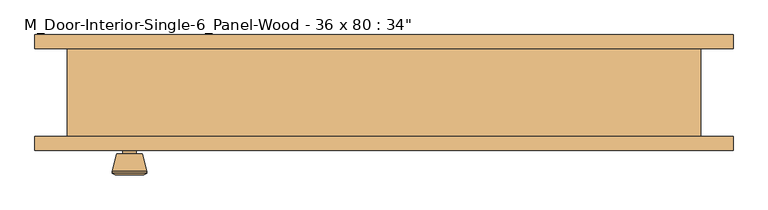
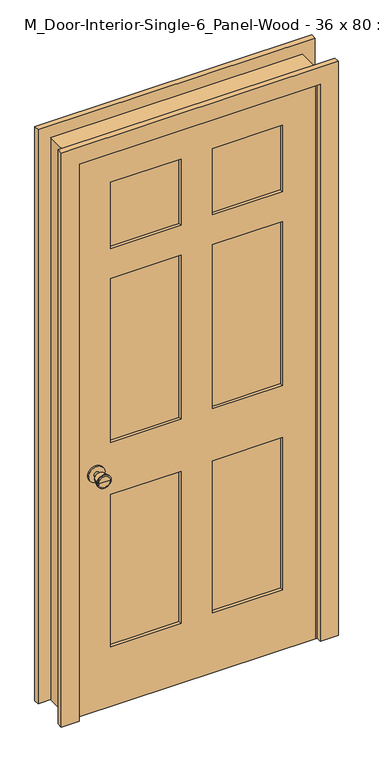
"""IFC4 building model written with IfcOpenShell, lengths in millimetres: door geometry."""

from ifc_helpers import new_model, si_unit, point, frame, frame_2d, origin, place, context, project, spatial, polyline, circle_curve, trimmed, segment, composite_curve, outline, extrude, faceted_brep, source, transform, mapped, element, save
from ifc_brep_helpers import plane_surface, cylinder_surface, revolved_surface, advanced_brep


def door_84de55a3(model_context):
    return source(origin(), model_context, "Body", "SolidModel", [
        advanced_brep(
        [(-366.8, -19.325, 914.4), (-376.8, -19.325, 914.4), (-356.8, -19.325, 914.4), (-346.3241324, 29.675, 914.4), (-387.2758676, 29.675, 914.4), (-366.8, 29.675, 914.4), (-341.8, 27.8471319, 914.4), (-391.8, 27.8471319, 914.4), (-341.8, 24.3834537, 914.4), (-391.8, 24.3834537, 914.4), (-348.163764, -0.325, 914.4), (-385.436236, -0.325, 914.4), (-356.8, -0.325, 914.4), (-376.8, -0.325, 914.4)],
        [
            (0, 1),
            (1, 2, circle_curve(frame((-366.8, -19.325, 914.4), z_axis=(0.0, -1.0, 0.0), x_axis=(-1.0, 0.0, 0.0)), 10.0)),
            (2, 0),
            (2, 1, circle_curve(frame((-366.8, -19.325, 914.4), z_axis=(0.0, -1.0, 0.0), x_axis=(-1.0, 0.0, 0.0)), 10.0)),
            (3, 4, circle_curve(frame((-366.8, 29.675, 914.4), z_axis=(0.0, 1.0, 0.0), x_axis=(-1.0, 0.0, 0.0)), 20.4758676)),
            (4, 5),
            (5, 3),
            (4, 3, circle_curve(frame((-366.8, 29.675, 914.4), z_axis=(0.0, 1.0, 0.0), x_axis=(-1.0, 0.0, 0.0)), 20.4758676)),
            (6, 7, circle_curve(frame((-366.8, 27.8471319, 914.4), z_axis=(0.0, 1.0, 0.0), x_axis=(-1.0, 0.0, 0.0)), 25.0)),
            (7, 4),
            (3, 6),
            (7, 6, circle_curve(frame((-366.8, 27.8471319, 914.4), z_axis=(0.0, 1.0, 0.0), x_axis=(-1.0, 0.0, 0.0)), 25.0)),
            (8, 9, circle_curve(frame((-366.8, 24.3834537, 914.4), z_axis=(0.0, 1.0, 0.0), x_axis=(-1.0, 0.0, 0.0)), 25.0)),
            (9, 7),
            (6, 8),
            (9, 8, circle_curve(frame((-366.8, 24.3834537, 914.4), z_axis=(0.0, 1.0, 0.0), x_axis=(-1.0, 0.0, 0.0)), 25.0)),
            (10, 11, circle_curve(frame((-366.8, -0.325, 914.4), z_axis=(0.0, 1.0, 0.0), x_axis=(-1.0, 0.0, 0.0)), 18.636236)),
            (11, 9),
            (8, 10),
            (11, 10, circle_curve(frame((-366.8, -0.325, 914.4), z_axis=(0.0, 1.0, 0.0), x_axis=(-1.0, 0.0, 0.0)), 18.636236)),
            (12, 13, circle_curve(frame((-366.8, -0.325, 914.4), z_axis=(0.0, 1.0, 0.0), x_axis=(-1.0, 0.0, 0.0)), 10.0)),
            (13, 11),
            (10, 12),
            (13, 12, circle_curve(frame((-366.8, -0.325, 914.4), z_axis=(0.0, 1.0, 0.0), x_axis=(-1.0, 0.0, 0.0)), 10.0)),
            (1, 13),
            (12, 2),
        ],
        [
            plane_surface(frame((-366.8, -19.325, 914.4), z_axis=(0.0, -1.0, 0.0), x_axis=(-1.0, 0.0, 0.0))),
            plane_surface(frame((-366.8, 29.675, 914.4), z_axis=(0.0, 1.0, 0.0), x_axis=(-1.0, 0.0, 0.0))),
            revolved_surface(polyline([(-387.2758676, 29.675, 914.4), (-391.8, 27.8471319, 914.4)]), (-366.8, -19.325, 914.4), (0.0, -1.0, 0.0)),
            cylinder_surface(frame((-366.8, -19.325, 914.4), z_axis=(0.0, -1.0, 0.0), x_axis=(-1.0, 0.0, 0.0)), 25.0),
            revolved_surface(polyline([(-391.8, 24.3834537, 914.4), (-385.436236, -0.325, 914.4)]), (-366.8, -19.325, 914.4), (0.0, -1.0, 0.0)),
            plane_surface(frame((-366.8, -0.325, 914.4), z_axis=(0.0, -1.0, 0.0), x_axis=(-1.0, 0.0, 0.0))),
            cylinder_surface(frame((-366.8, -19.325, 914.4), z_axis=(0.0, -1.0, 0.0), x_axis=(-1.0, 0.0, 0.0)), 10.0),
        ],
        [
            (0, [[1, 2, 3]]),
            (0, [[-3, 4, -1]]),
            (1, [[5, 6, 7]]),
            (1, [[8, -7, -6]]),
            (2, [[9, 10, -5, 11]]),
            (2, [[12, -11, -8, -10]]),
            (3, [[13, 14, -9, 15]]),
            (3, [[16, -15, -12, -14]]),
            (4, [[17, 18, -13, 19]]),
            (4, [[20, -19, -16, -18]]),
            (5, [[21, 22, -17, 23]]),
            (5, [[24, -23, -20, -22]]),
            (6, [[-2, 25, -21, 26]]),
            (6, [[-4, -26, -24, -25]]),
        ],
    ),
        extrude(outline(composite_curve([segment(trimmed(circle_curve(frame_2d((914.4, -366.8)), 30.0), [point((914.4, -396.8))], [point((914.4, -336.8))], False, "CARTESIAN"), True, "CONTINUOUS"), segment(trimmed(circle_curve(frame_2d((914.4, -366.8)), 30.0), [point((914.4, -336.8))], [point((914.4, -396.8))], False, "CARTESIAN"), True, "CONTINUOUS")], self_intersect=False)), frame((0.0, -25.325, 0.0), z_axis=(0.0, 1.0, 0.0), x_axis=(0.0, 0.0, 1.0)), (0.0, 0.0, 1.0), 6.0),
        advanced_brep(
        [(-366.8, -66.325, 914.4), (-356.8, -66.325, 914.4), (-376.8, -66.325, 914.4), (-346.3241324, -115.325, 914.4), (-366.8, -115.325, 914.4), (-387.2758676, -115.325, 914.4), (-341.8, -113.4971319, 914.4), (-391.8, -113.4971319, 914.4), (-341.8, -110.0334537, 914.4), (-391.8, -110.0334537, 914.4), (-348.163764, -85.325, 914.4), (-385.436236, -85.325, 914.4), (-356.8, -85.325, 914.4), (-376.8, -85.325, 914.4)],
        [
            (0, 1),
            (1, 2, circle_curve(frame((-366.8, -66.325, 914.4), z_axis=(0.0, 1.0, 0.0), x_axis=(-1.0, 0.0, 0.0)), 10.0)),
            (2, 0),
            (2, 1, circle_curve(frame((-366.8, -66.325, 914.4), z_axis=(0.0, 1.0, 0.0), x_axis=(-1.0, 0.0, 0.0)), 10.0)),
            (3, 4),
            (4, 5),
            (5, 3, circle_curve(frame((-366.8, -115.325, 914.4), z_axis=(0.0, -1.0, 0.0), x_axis=(-1.0, 0.0, 0.0)), 20.4758676)),
            (3, 5, circle_curve(frame((-366.8, -115.325, 914.4), z_axis=(0.0, -1.0, 0.0), x_axis=(-1.0, 0.0, 0.0)), 20.4758676)),
            (6, 3),
            (5, 7),
            (7, 6, circle_curve(frame((-366.8, -113.4971319, 914.4), z_axis=(0.0, -1.0, 0.0), x_axis=(-1.0, 0.0, 0.0)), 25.0)),
            (6, 7, circle_curve(frame((-366.8, -113.4971319, 914.4), z_axis=(0.0, -1.0, 0.0), x_axis=(-1.0, 0.0, 0.0)), 25.0)),
            (8, 6),
            (7, 9),
            (9, 8, circle_curve(frame((-366.8, -110.0334537, 914.4), z_axis=(0.0, -1.0, 0.0), x_axis=(-1.0, 0.0, 0.0)), 25.0)),
            (8, 9, circle_curve(frame((-366.8, -110.0334537, 914.4), z_axis=(0.0, -1.0, 0.0), x_axis=(-1.0, 0.0, 0.0)), 25.0)),
            (10, 8),
            (9, 11),
            (11, 10, circle_curve(frame((-366.8, -85.325, 914.4), z_axis=(0.0, -1.0, 0.0), x_axis=(-1.0, 0.0, 0.0)), 18.636236)),
            (10, 11, circle_curve(frame((-366.8, -85.325, 914.4), z_axis=(0.0, -1.0, 0.0), x_axis=(-1.0, 0.0, 0.0)), 18.636236)),
            (12, 10),
            (11, 13),
            (13, 12, circle_curve(frame((-366.8, -85.325, 914.4), z_axis=(0.0, -1.0, 0.0), x_axis=(-1.0, 0.0, 0.0)), 10.0)),
            (12, 13, circle_curve(frame((-366.8, -85.325, 914.4), z_axis=(0.0, -1.0, 0.0), x_axis=(-1.0, 0.0, 0.0)), 10.0)),
            (1, 12),
            (13, 2),
        ],
        [
            plane_surface(frame((-366.8, -66.325, 914.4), z_axis=(0.0, 1.0, 0.0), x_axis=(-1.0, 0.0, 0.0))),
            plane_surface(frame((-366.8, -115.325, 914.4), z_axis=(0.0, -1.0, 0.0), x_axis=(-1.0, 0.0, 0.0))),
            revolved_surface(polyline([(-387.2758676, -115.325, 914.4), (-391.8, -113.4971319, 914.4)]), (-366.8, -66.325, 914.4), (0.0, 1.0, 0.0)),
            cylinder_surface(frame((-366.8, -66.325, 914.4), z_axis=(0.0, 1.0, 0.0), x_axis=(-1.0, 0.0, 0.0)), 25.0),
            revolved_surface(polyline([(-391.8, -110.0334537, 914.4), (-385.436236, -85.325, 914.4)]), (-366.8, -66.325, 914.4), (0.0, 1.0, 0.0)),
            plane_surface(frame((-366.8, -85.325, 914.4), z_axis=(0.0, 1.0, 0.0), x_axis=(-1.0, 0.0, 0.0))),
            cylinder_surface(frame((-366.8, -66.325, 914.4), z_axis=(0.0, 1.0, 0.0), x_axis=(-1.0, 0.0, 0.0)), 10.0),
        ],
        [
            (0, [[1, 2, 3]]),
            (0, [[-3, 4, -1]]),
            (1, [[5, 6, 7]]),
            (1, [[-6, -5, 8]]),
            (2, [[9, -7, 10, 11]]),
            (2, [[-10, -8, -9, 12]]),
            (3, [[13, -11, 14, 15]]),
            (3, [[-14, -12, -13, 16]]),
            (4, [[17, -15, 18, 19]]),
            (4, [[-18, -16, -17, 20]]),
            (5, [[21, -19, 22, 23]]),
            (5, [[-22, -20, -21, 24]]),
            (6, [[25, -23, 26, -2]]),
            (6, [[-26, -24, -25, -4]]),
        ],
    ),
        extrude(outline(composite_curve([segment(trimmed(circle_curve(frame_2d((914.4, -366.8)), 30.0), [point((914.4, -396.8))], [point((914.4, -336.8))], False, "CARTESIAN"), True, "CONTINUOUS"), segment(trimmed(circle_curve(frame_2d((914.4, -366.8)), 30.0), [point((914.4, -336.8))], [point((914.4, -396.8))], False, "CARTESIAN"), True, "CONTINUOUS")], self_intersect=False)), frame((0.0, -66.325, 0.0), z_axis=(0.0, 1.0, 0.0), x_axis=(0.0, 0.0, 1.0)), (0.0, 0.0, 1.0), 6.0),
        extrude(outline(polyline([(311.8, -36.9916667), (311.8, -48.6583333), (57.5, -48.6583333), (57.5, -36.9916667), (311.8, -36.9916667)])), frame((0.0, 0.0, 1759.3), z_axis=(0.0, 0.0, 1.0), x_axis=(1.0, 0.0, 0.0)), (0.0, 0.0, 1.0), 254.3),
        extrude(outline(polyline([(311.8, -36.9916667), (311.8, -48.6583333), (57.5, -48.6583333), (57.5, -36.9916667), (311.8, -36.9916667)])), frame((0.0, 0.0, 1014.4), z_axis=(0.0, 0.0, 1.0), x_axis=(1.0, 0.0, 0.0)), (0.0, 0.0, 1.0), 629.9),
        extrude(outline(polyline([(-57.5, -36.9916667), (-57.5, -48.6583333), (-311.8, -48.6583333), (-311.8, -36.9916667), (-57.5, -36.9916667)])), frame((0.0, 0.0, 1014.4), z_axis=(0.0, 0.0, 1.0), x_axis=(1.0, 0.0, 0.0)), (0.0, 0.0, 1.0), 629.9),
        extrude(outline(polyline([(-57.5, -36.9916667), (-57.5, -48.6583333), (-311.8, -48.6583333), (-311.8, -36.9916667), (-57.5, -36.9916667)])), frame((0.0, 0.0, 1759.3), z_axis=(0.0, 0.0, 1.0), x_axis=(1.0, 0.0, 0.0)), (0.0, 0.0, 1.0), 254.3),
        extrude(outline(polyline([(311.8, -36.9916667), (311.8, -48.6583333), (57.5, -48.6583333), (57.5, -36.9916667), (311.8, -36.9916667)])), frame((0.0, 0.0, 230.0), z_axis=(0.0, 0.0, 1.0), x_axis=(1.0, 0.0, 0.0)), (0.0, 0.0, 1.0), 584.4),
        extrude(outline(polyline([(-57.5, -36.9916667), (-57.5, -48.6583333), (-311.8, -48.6583333), (-311.8, -36.9916667), (-57.5, -36.9916667)])), frame((0.0, 0.0, 230.0), z_axis=(0.0, 0.0, 1.0), x_axis=(1.0, 0.0, 0.0)), (0.0, 0.0, 1.0), 584.4),
        extrude(outline(polyline([(2133.6, -431.8), (0.0, -431.8), (0.0, 431.8), (2133.6, 431.8), (2133.6, -431.8)]), holes=[polyline([(2013.6, 57.5), (2013.6, 311.8), (1759.3, 311.8), (1759.3, 57.5), (2013.6, 57.5)]), polyline([(1644.3, 311.8), (1014.4, 311.8), (1014.4, 57.5), (1644.3, 57.5), (1644.3, 311.8)]), polyline([(1014.4, -57.5), (1014.4, -311.8), (1644.3, -311.8), (1644.3, -57.5), (1014.4, -57.5)]), polyline([(1759.3, -311.8), (2013.6, -311.8), (2013.6, -57.5), (1759.3, -57.5), (1759.3, -311.8)]), polyline([(814.4, 57.5), (814.4, 311.8), (230.0, 311.8), (230.0, 57.5), (814.4, 57.5)]), polyline([(230.0, -57.5), (230.0, -311.8), (814.4, -311.8), (814.4, -57.5), (230.0, -57.5)])]), frame((0.0, -60.325, 0.0), z_axis=(0.0, 1.0, 0.0), x_axis=(0.0, 0.0, 1.0)), (0.0, 0.0, 1.0), 35.0),
        faceted_brep([(456.8, -60.325, 0.0), (431.8, -60.325, 0.0), (431.8, -25.325, 0.0), (419.1, -25.325, 0.0), (419.1, 9.6, 0.0), (431.8, 9.6, 0.0), (431.8, 66.675, 0.0), (456.8, 66.675, 0.0), (456.8, 66.675, 2158.6), (456.8, -60.325, 2158.6), (431.8, 66.675, 2133.6), (-431.8, 66.675, 2133.6), (-431.8, 66.675, 0.0), (-456.8, 66.675, 0.0), (-456.8, 66.675, 2158.6), (431.8, 9.6, 2133.6), (419.1, 9.6, 2120.9), (-419.1, 9.6, 2120.9), (-419.1, 9.6, 0.0), (-431.8, 9.6, 0.0), (-431.8, 9.6, 2133.6), (419.1, -25.325, 2120.9), (431.8, -25.325, 2133.6), (-431.8, -25.325, 2133.6), (-431.8, -25.325, 0.0), (-419.1, -25.325, 0.0), (-419.1, -25.325, 2120.9), (431.8, -60.325, 2133.6), (-456.8, -60.325, 2158.6), (-456.8, -60.325, 0.0), (-431.8, -60.325, 0.0), (-431.8, -60.325, 2133.6)], [[[0, 1, 2, 3, 4, 5, 6, 7]], [[7, 8, 9, 0]], [[6, 10, 11, 12, 13, 14, 8, 7]], [[5, 15, 10, 6]], [[4, 16, 17, 18, 19, 20, 15, 5]], [[3, 21, 16, 4]], [[2, 22, 23, 24, 25, 26, 21, 3]], [[1, 27, 22, 2]], [[0, 9, 28, 29, 30, 31, 27, 1]], [[8, 14, 28, 9]], [[15, 20, 11, 10]], [[21, 26, 17, 16]], [[27, 31, 23, 22]], [[29, 13, 12, 19, 18, 25, 24, 30]], [[14, 13, 29, 28]], [[20, 19, 12, 11]], [[26, 25, 18, 17]], [[31, 30, 24, 23]]]),
        extrude(outline(polyline([(0.0, 503.15), (2204.95, 503.15), (2204.95, -503.15), (0.0, -503.15), (0.0, -438.15), (2139.95, -438.15), (2139.95, 438.15), (0.0, 438.15), (0.0, 503.15)])), frame((0.0, 66.675, 0.0), z_axis=(0.0, 1.0, 0.0), x_axis=(0.0, 0.0, 1.0)), (0.0, 0.0, 1.0), 20.0),
        extrude(outline(polyline([(0.0, 503.15), (2204.95, 503.15), (2204.95, -503.15), (0.0, -503.15), (0.0, -438.15), (2139.95, -438.15), (2139.95, 438.15), (0.0, 438.15), (0.0, 503.15)])), frame((0.0, -80.325, 0.0), z_axis=(0.0, 1.0, 0.0), x_axis=(0.0, 0.0, 1.0)), (0.0, 0.0, 1.0), 20.0),
    ])


if __name__ == "__main__":
    model = new_model("IFC4")
    model_context = context("Model", 3, world=origin())
    ifc_project = project(units=[si_unit("LENGTHUNIT", "METRE", prefix="MILLI")], contexts=[model_context])
    site = spatial("IfcSite", under=ifc_project)
    building = spatial("IfcBuilding", under=site)
    placement = place(None, origin())
    door_shape = door_84de55a3(model_context)
    element("IfcDoor", 1, ObjectType="M_Door-Interior-Single-6_Panel-Wood - 36 x 80 : 34\"", at=placement, inside=building, context=model_context, shape_type="MappedRepresentation", body=[
        mapped(door_shape, transform((0.0, 0.0, 0.0), x_axis=(1.0, 0.0, 0.0), y_axis=(0.0, 1.0, 0.0), z_axis=(0.0, 0.0, 1.0))),
    ])
    save(model, "model.ifc")

# Revit data of these elements
# Type "M_Door-Interior-Single-6_Panel-Wood - 36 x 80 : 34\""
#   Type Mark = "t"
#   Assembly Code = "C1020300"
#   Analytic Construction = "Wooden"
#   Top Rail = 0' - 4.72441"
#   Top Panel = 0' - 10.01181"
#   Thickness = 0' - 1.37795"
#   Thermal Resistance (R) = 0.455703 (m²·K)/W
#   Swing Angle [instance default] = 90.00°
#   Stiles = 0' - 4.72441"
#   Rough Width = 2' - 11.9685"
#   Rough Height = 7' - 0.98425"
#   Mullion = 0' - 4.52756"
#   Lock Rail = 0' - 7.87402"
#   Intermediate Rail = 0' - 4.52756"
#   Height = 7' - 0"
#   Width = 2' - 10"
#   Heat Transfer Coefficient (U) = 2.19465 W/(m²·K)
#   Bottom Rail = 0' - 9.05512"
#   Trim Material = Trim
#   Panel Material = Trim
#   Frame Material = Trim
#   Door Handle Material = Aluminum
#   Visual Light Transmittance = 0
#   Solar Heat Gain Coefficient = 0
#   Wall Closure = (empty or 0)
#   Function = (empty or 0)
# Element 1 (IfcDoor, "M_Door-Interior-Single-6_Panel-Wood - 36 x 80 : 34\"")
#   Materials on its faces: "Trim", "Aluminum"
# Materials
#   "Trim": class "Wood", colour RGB 250 251 245, transparency 0, Cost = 0
#   "Aluminum": class "Metal", colour RGB 244 244 244, transparency 0, Description = "Aluminum 6061", Cost = 0
